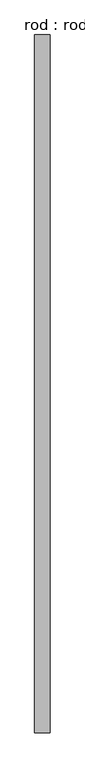
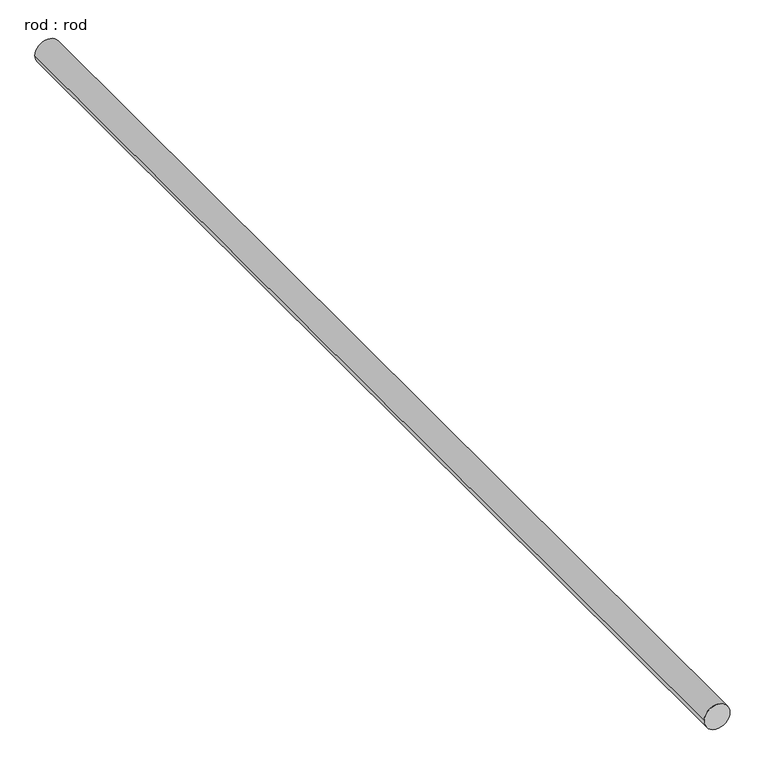
"""IFC4 building model written with IfcOpenShell, lengths in millimetres: proxy geometry, rod : rod."""

from ifc_helpers import new_model, si_unit, point, frame, frame_2d, origin, place, context, project, spatial, circle_curve, trimmed, segment, composite_curve, outline, extrude, source, transform, mapped, element, save


def rod_rod_32baba29(model_context):
    return source(origin(), model_context, "Body", "SweptSolid", [
        extrude(outline(composite_curve([segment(trimmed(circle_curve(frame_2d((0.0108462, 0.0)), 200.0), [point((0.0108462, 200.0))], [point((0.0108462, -200.0))], False, "CARTESIAN"), True, "CONTINUOUS"), segment(trimmed(circle_curve(frame_2d((0.0108462, 0.0)), 200.0), [point((0.0108462, -200.0))], [point((0.0108462, 200.0))], False, "CARTESIAN"), True, "CONTINUOUS")], self_intersect=False)), frame((0.0, -4907.2713847, 0.0), z_axis=(0.0, 1.0, 0.0), x_axis=(0.0, 0.0, 1.0)), (0.0, 0.0, 1.0), 18000.0),
    ])


if __name__ == "__main__":
    model = new_model("IFC4")
    model_context = context("Model", 3, world=origin())
    ifc_project = project(units=[si_unit("LENGTHUNIT", "METRE", prefix="MILLI")], contexts=[model_context])
    site = spatial("IfcSite", under=ifc_project)
    building = spatial("IfcBuilding", under=site)
    placement = place(None, origin())
    rod_rod_shape = rod_rod_32baba29(model_context)
    element("IfcBuildingElementProxy", 1, Name="rod : rod", ObjectType="rod : rod", at=placement, inside=building, context=model_context, shape_type="MappedRepresentation", body=[
        mapped(rod_rod_shape, transform((0.0, 0.0, 0.0), x_axis=(1.0, 0.0, 0.0), y_axis=(0.0, 1.0, 0.0), z_axis=(0.0, 0.0, 1.0))),
    ])
    save(model, "model.ifc")

# Revit data of these elements
# Type "rod : rod"
#   Default Elevation = 0
